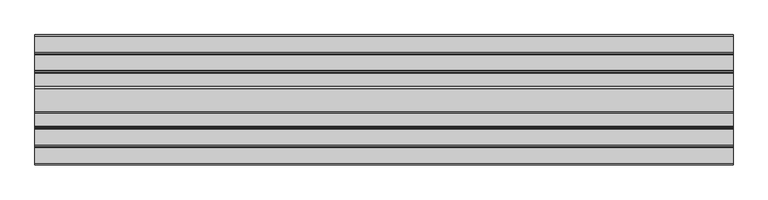
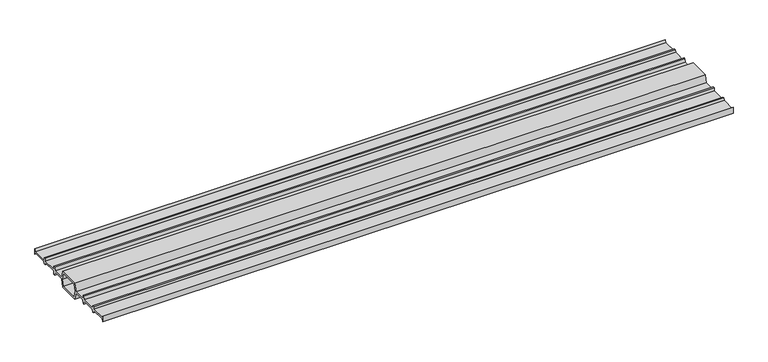
"""IFC4 building model written with IfcOpenShell, lengths in millimetres: proxy geometry, TN_Гидрошпонка ТН Фундамент : Гидрошпонка ТН Фундамент ДШ-В-280."""

from ifc_helpers import new_model, si_unit, frame, origin, place, context, project, spatial, polyline, outline, extrude, source, transform, mapped, element, save


def specialty_equipment_ce665a1a(model_context):
    return source(origin(), model_context, "Body", "SweptSolid", [
        extrude(outline(polyline([(-98.280218, -5.7544352), (-101.719782, -5.7544352), (-102.7344441, 0.0), (-136.5809483, 0.0), (-140.0, -5.5044352), (-140.0, 9.4955648), (-136.5809483, 3.9911296), (-102.7344441, 3.9911296), (-101.719782, 9.7455648), (-98.280218, 9.7455648), (-97.2655559, 3.9911296), (-63.0288318, 3.9911296), (-61.7513068, 11.75), (-58.2486932, 11.75), (-56.9722041, 3.9974211), (-29.5057388, 3.9974211), (-24.730127, 21.8202469), (24.730127, 21.8202469), (29.5057388, 3.9974211), (56.9722041, 3.9974211), (58.2486932, 11.75), (61.7513068, 11.75), (63.0288318, 3.9911296), (97.2655559, 3.9911296), (98.280218, 9.7455648), (101.719782, 9.7455648), (102.7344441, 3.9911296), (136.5809483, 3.9911296), (140.0, 9.4955648), (140.0, -5.5044352), (136.5809483, 0.0), (102.7344441, 0.0), (101.719782, -5.7544352), (98.280218, -5.7544352), (97.2655559, 0.0), (63.1139579, 0.0), (61.7513068, -8.2758715), (58.2486932, -8.2758715), (56.8860421, 0.0), (29.5057388, 0.0), (24.730127, -17.8228258), (-24.730127, -17.8228258), (-29.5057388, 0.0), (-56.8860421, 0.0), (-58.2486932, -8.2758715), (-61.7513068, -8.2758715), (-63.1139579, 0.0), (-97.2655559, 0.0), (-98.280218, -5.7544352)]), holes=[polyline([(-24.9720905, 2.3987105), (-20.8934921, -12.8228258), (20.8934921, -12.8228258), (24.9720905, 2.3987105), (21.1078514, 16.8202469), (-21.1078514, 16.8202469), (-24.9720905, 2.3987105)])]), frame((0.0115641, 0.0, 0.0), z_axis=(1.0, 0.0, 0.0), x_axis=(0.0, 1.0, 0.0)), (0.0, 0.0, 1.0), 1500.0),
    ])


if __name__ == "__main__":
    model = new_model("IFC4")
    model_context = context("Model", 3, world=origin())
    ifc_project = project(units=[si_unit("LENGTHUNIT", "METRE", prefix="MILLI")], contexts=[model_context])
    site = spatial("IfcSite", under=ifc_project)
    building = spatial("IfcBuilding", under=site)
    placement = place(None, origin())
    specialty_equipment_shape = specialty_equipment_ce665a1a(model_context)
    element("IfcBuildingElementProxy", 1, Name="TN_Гидрошпонка ТН Фундамент : Гидрошпонка ТН Фундамент ДШ-В-280", ObjectType="TN_Гидрошпонка ТН Фундамент : Гидрошпонка ТН Фундамент ДШ-В-280", at=placement, inside=building, context=model_context, shape_type="MappedRepresentation", body=[
        mapped(specialty_equipment_shape, transform((0.0, 0.0, 0.0), x_axis=(1.0, 0.0, 0.0), y_axis=(0.0, 1.0, 0.0), z_axis=(0.0, 0.0, 1.0))),
    ])
    save(model, "model.ifc")

# Revit data of these elements
# Type "TN_Гидрошпонка ТН Фундамент : Гидрошпонка ТН Фундамент ДШ-В-280"
#   Description = "Внутренние гидроизоляционные шпонки ТН Фундамент ДШ-В предназначены для герметизации деформационных швов бетонирования при строительстве подземных и заглубленных конструкций зданий и сооружений различного назначения и класса ответственности."
#   Type Comments = "п.м."
#   Manufacturer = "ТехноНИКОЛЬ"
#   URL = "https://nav.tn.ru/catalog/gidroizolyatsiya/komplektatsiya-dlya-gidroizolyatsii/gidroshponki-tekhnonikol-fundament-dsh-v/"
#   ADSK_Примечание = ""
#   ADSK_Обозначение [instance default] = "ТехноНИКОЛЬ"
#   ADSK_Наименование = "Гидрошпонка ТН Фундамент ДШ-В-280"
#   ADSK_Масса_Текст = ""
#   ADSK_Марка = ""
#   ADSK_Код изделия = "66670"
#   ADSK_Завод-изготовитель [instance default] = "ТехноНИКОЛЬ"
#   ADSK_Единица измерения [instance default] = "п.м."
#   ADSK_Группирование = "Гидрошпонки"
#   ADSK_URL страницы изделия = "https://nav.tn.ru/catalog/gidroizolyatsiya/komplektatsiya-dlya-gidroizolyatsii/gidroshponki-tekhnonikol-fundament-dsh-v/"
#   ADSK_URL документации изделия = "https://nav.tn.ru/upload/iblock/28f/fdn3hm8k6c3nnk1qf6d2lbujw61o7ba5/Tekhlist-7.398_Gidroshponki-TN-Fundament-DSH_V_RU_ru.pdf"
#   built-in parameter 1001306 [instance default] = 3.28084 (stored number, unit not read)
#   ADSK_Размер_Длина [instance default] = 1000 mm
#   ADSK_Количество [instance default] = 1
#   Гидрошпонка ТН Фундамент ТШ-Н-210 = no
#   Гидрошпонка ТН Фундамент ДШП-В-50 = no
#   Гидрошпонка ТН Фундамент ДШП-В-20 = no
#   Гидрошпонка ТН Фундамент ДШ-В-280 = yes
#   Гидрошпонка ТН Фундамент ДШ-В-250 = no
#   Гидрошпонка ТН Фундамент ТШ-В-250 = no
#   Гидрошпонка ТН Фундамент ТПС-В 140-1 = no
#   Гидрошпонка ТН Фундамент ДШ-Н-280 = no
#   Гидрошпонка ТН Фундамент ДШ-Н-250 = no
#   Гидрошпонка ТН Фундамент ТПС-В 100-2 = no
#   Гидрошпонка ТН Фундамент ТШ-Н-250 = no
#   Гидрошпонка ТН Фундамент ТШ-В-210 = no
#   Материал = TN_ПВХ_Черный
#   Default Elevation = 0
# Element 1 (IfcBuildingElementProxy, "TN_Гидрошпонка ТН Фундамент : Гидрошпонка ТН Фундамент ДШ-В-280")
#   built-in parameter 1001306 = 4.92126 (stored number, unit not read)
#   ADSK_Размер_Длина = 1500 mm
#   ADSK_Количество = 1.5
#   Materials on its faces: "TN_ПВХ_Черный"
# Materials
#   "TN_ПВХ_Черный": class "Типовые", colour RGB 48 48 48, transparency 0, Cost = 0
